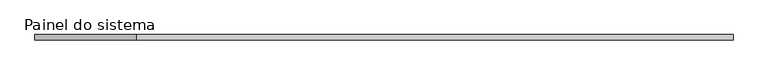
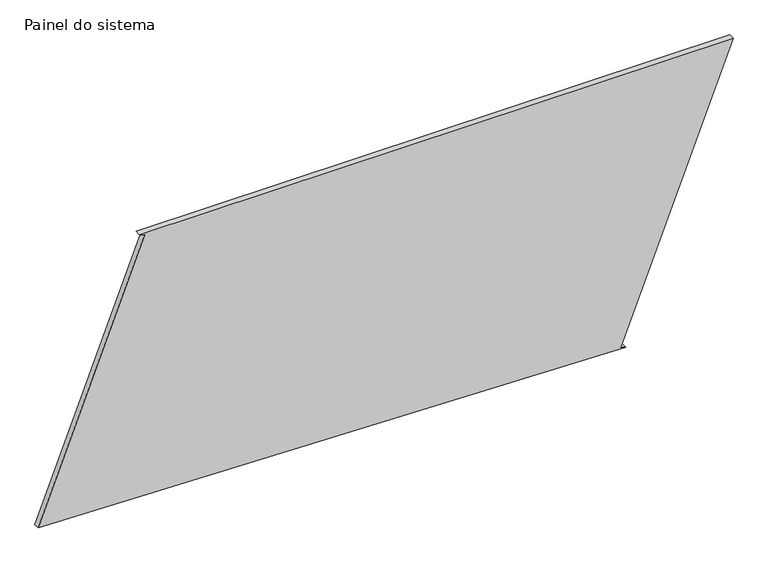
"""IFC4 building model written with IfcOpenShell, lengths in millimetres: plate geometry, Painel do sistema : Envidraçado."""

import ifcopenshell
import ifcopenshell.guid

model = None  # the IFC model being written
_history = None  # IfcOwnerHistory: only IFC2X3 demands one
_inside = {}  # id of a spatial element -> (the spatial element, [elements in it])
_under = {}  # id of a project, library or spatial element -> (it, [spatial elements below it])
_declared = {}  # id of a project -> (the project, [libraries it declares])
_typed = {}  # id of a type object -> (the type object, [elements of that type])
_made_of = {}  # id of a material, layer set ... -> (it, [elements and type objects made of it])


def new_model(schema):
    """Start an empty IFC model of exactly this schema.

    Asked for "IFC4X3", IfcOpenShell would pick the latest addendum, in which some entities
    have other attributes; the version numbers below select the first issue.
    IFC2X3 requires an IfcOwnerHistory on every rooted entity: one is made here for all.
    """
    global model, _history
    if schema == "IFC4X3":
        model = ifcopenshell.file(schema_version=(4, 3, 0, 0))
    else:
        model = ifcopenshell.file(schema=schema)
    _inside.clear()
    _under.clear()
    _declared.clear()
    _typed.clear()
    _made_of.clear()
    _history = None
    if model.schema == "IFC2X3":
        org = make("IfcOrganization", Name="unknown")
        user = make(
            "IfcPersonAndOrganization",
            ThePerson=make("IfcPerson", FamilyName="unknown"),
            TheOrganization=org,
        )
        app = make(
            "IfcApplication",
            ApplicationDeveloper=org,
            Version="unknown",
            ApplicationFullName="unknown",
            ApplicationIdentifier="unknown",
        )
        _history = make(
            "IfcOwnerHistory",
            OwningUser=user,
            OwningApplication=app,
            ChangeAction="ADDED",
            CreationDate=0,
        )
    return model


def make(cls, **values):
    """One entity of the class cls with the attributes given. An attribute that is None is left unset."""
    return model.create_entity(
        cls, **{name: value for name, value in values.items() if value is not None}
    )


def rooted(cls, **values):
    """An entity with a GlobalId (a new one), such as an element, a storey or a relation."""
    return make(cls, GlobalId=ifcopenshell.guid.new(), OwnerHistory=_history, **values)


def si_unit(unit_type, name, prefix=None):
    """IfcSIUnit, for example si_unit("LENGTHUNIT", "METRE", prefix="MILLI")."""
    return make("IfcSIUnit", UnitType=unit_type, Prefix=prefix, Name=name)


def assignment(units):
    """IfcUnitAssignment: the units of a project."""
    return None if units is None else make("IfcUnitAssignment", Units=units)


def point(xyz):
    """IfcCartesianPoint."""
    return None if xyz is None else make("IfcCartesianPoint", Coordinates=xyz)


def direction(xyz):
    """IfcDirection."""
    return None if xyz is None else make("IfcDirection", DirectionRatios=xyz)


def frame(location, z_axis=None, x_axis=None):
    """IfcAxis2Placement3D, a coordinate frame: its origin and axes. An axis left out is left unset."""
    return make(
        "IfcAxis2Placement3D",
        Location=point(location),
        Axis=direction(z_axis),
        RefDirection=direction(x_axis),
    )


def origin():
    """The frame at (0, 0, 0) with its axes left unset."""
    return frame((0.0, 0.0, 0.0))


def place(relative_to, where):
    """IfcLocalPlacement: puts the frame where relative to a parent placement (None: the world)."""
    return make(
        "IfcLocalPlacement", PlacementRelTo=relative_to, RelativePlacement=where
    )


def context(
    kind, dimensions, precision=None, world=None, true_north=None, identifier=None
):
    """IfcGeometricRepresentationContext, for example the 3D "Model" context."""
    return make(
        "IfcGeometricRepresentationContext",
        ContextIdentifier=identifier,
        ContextType=kind,
        CoordinateSpaceDimension=dimensions,
        Precision=precision,
        WorldCoordinateSystem=world,
        TrueNorth=true_north,
    )


def project(units=None, contexts=None):
    """IfcProject with its units and contexts."""
    return rooted(
        "IfcProject",
        Name="project",
        RepresentationContexts=contexts,
        UnitsInContext=assignment(units),
    )


def spatial(cls, under=None, at=None, **own):
    """A site, building, storey or space (cls), placed at a placement, below another one or the project."""
    s = rooted(cls, ObjectPlacement=at, **own)
    if under is not None:
        _under.setdefault(under.id(), (under, []))[1].append(s)
    return s


def polyline(points):
    """IfcPolyline through the points."""
    return make("IfcPolyline", Points=[point(p) for p in points])


def outline(outer, holes=None, kind="AREA"):
    """IfcArbitraryClosedProfileDef: a profile drawn as a closed curve; with holes, ...WithVoids."""
    if holes is None:
        return make("IfcArbitraryClosedProfileDef", ProfileType=kind, OuterCurve=outer)
    return make(
        "IfcArbitraryProfileDefWithVoids",
        ProfileType=kind,
        OuterCurve=outer,
        InnerCurves=holes,
    )


def extrude(swept, where, along, depth):
    """IfcExtrudedAreaSolid: the profile swept, set in the frame where, extruded along a direction by depth."""
    return make(
        "IfcExtrudedAreaSolid",
        SweptArea=swept,
        Position=where,
        ExtrudedDirection=direction(along),
        Depth=depth,
    )


def shape(context_of_items, identifier, shape_type, items):
    """IfcShapeRepresentation: the items that make up one representation, for example the "Body"."""
    return make(
        "IfcShapeRepresentation",
        ContextOfItems=context_of_items,
        RepresentationIdentifier=identifier,
        RepresentationType=shape_type,
        Items=items,
    )


def source(mapping_origin, context_of_items, identifier, shape_type, items):
    """IfcRepresentationMap: a shape defined once, which mapped items show again and again."""
    return make(
        "IfcRepresentationMap",
        MappingOrigin=mapping_origin,
        MappedRepresentation=shape(context_of_items, identifier, shape_type, items),
    )


def transform(
    local_origin,
    x_axis=None,
    y_axis=None,
    z_axis=None,
    scale=None,
    scale2=None,
    scale3=None,
    uniform=True,
):
    """IfcCartesianTransformationOperator3D, or its non-uniform kind. x_axis, y_axis, z_axis: its Axis1, 2, 3."""
    if uniform:
        return make(
            "IfcCartesianTransformationOperator3D",
            Axis1=direction(x_axis),
            Axis2=direction(y_axis),
            LocalOrigin=point(local_origin),
            Scale=scale,
            Axis3=direction(z_axis),
        )
    return make(
        "IfcCartesianTransformationOperator3DnonUniform",
        Axis1=direction(x_axis),
        Axis2=direction(y_axis),
        LocalOrigin=point(local_origin),
        Scale=scale,
        Axis3=direction(z_axis),
        Scale2=scale2,
        Scale3=scale3,
    )


def mapped(mapping_source, mapping_target):
    """IfcMappedItem: shows the shape of a source again, moved by a transform."""
    return make(
        "IfcMappedItem", MappingSource=mapping_source, MappingTarget=mapping_target
    )


def made_of(thing, what):
    """Note that an element or type object is made of a material, layer set ...; save() writes the relation."""
    if what is not None:
        _made_of.setdefault(what.id(), (what, []))[1].append(thing)
    return thing


def element(
    cls,
    number,
    at=None,
    inside=None,
    cuts=None,
    type_object=None,
    material=None,
    context=None,
    identifier="Body",
    shape_type=None,
    held_by="IfcProductDefinitionShape",
    body=None,
    shapes=None,
    **own,
):
    """One element of the class cls, such as IfcWall. Its Tag is "e" and its number.

    at: its placement. inside: the storey or other place that contains it. cuts: it is an
    opening in that element (IfcRelVoidsElement). A single representation is given by context,
    identifier, shape_type and body (its items); several are given by shapes. held_by: the class
    of the entity that holds the representations. save() writes the other relations.
    """
    e = rooted(cls, Tag="e%d" % number, ObjectPlacement=at, **own)
    if body is not None:
        shapes = [shape(context, identifier, shape_type, body)]
    if shapes is not None:
        e.Representation = make(held_by, Representations=shapes)
    if inside is not None:
        _inside.setdefault(inside.id(), (inside, []))[1].append(e)
    if cuts is not None:
        rooted(
            "IfcRelVoidsElement", RelatingBuildingElement=cuts, RelatedOpeningElement=e
        )
    if type_object is not None:
        _typed.setdefault(type_object.id(), (type_object, []))[1].append(e)
    return made_of(e, material)


def aggregate(whole, parts):
    """IfcRelAggregates: a whole, such as a stair, and the parts it consists of."""
    return rooted("IfcRelAggregates", RelatingObject=whole, RelatedObjects=parts)


def save(model, path):
    """Write the relations noted so far, then the file.

    IfcRelAggregates (storeys below a building ...), IfcRelContainedInSpatialStructure (elements
    in a storey), IfcRelDefinesByType, IfcRelAssociatesMaterial and IfcRelDeclares: one each for
    every whole, place, type object, material and project.
    """
    for whole, parts in _under.values():
        aggregate(whole, parts)
    for where, things in _inside.values():
        rooted(
            "IfcRelContainedInSpatialStructure",
            RelatedElements=things,
            RelatingStructure=where,
        )
    for kind, things in _typed.values():
        rooted("IfcRelDefinesByType", RelatedObjects=things, RelatingType=kind)
    for what, things in _made_of.values():
        rooted("IfcRelAssociatesMaterial", RelatedObjects=things, RelatingMaterial=what)
    for by, libraries in _declared.values():
        rooted("IfcRelDeclares", RelatingContext=by, RelatedDefinitions=libraries)
    model.write(path)


def painel_do_sistema_89789c02(model_context):
    return source(origin(), model_context, "Body", "SweptSolid", [
        extrude(outline(polyline([(0.0, 1107.0608873), (9.0972802, 1083.7748509), (1333.7866514, 1601.2983243), (1333.7866514, -1133.8482806), (1324.6893712, -1110.5622442), (68.5668902, -1601.2983243), (0.0, 1107.0608873)])), frame((0.0, 24.5, 0.0), z_axis=(0.0, 1.0, 0.0), x_axis=(0.0, 0.0, 1.0)), (0.0, 0.0, 1.0), 25.0),
    ])


if __name__ == "__main__":
    model = new_model("IFC4")
    model_context = context("Model", 3, world=origin())
    ifc_project = project(units=[si_unit("LENGTHUNIT", "METRE", prefix="MILLI")], contexts=[model_context])
    site = spatial("IfcSite", under=ifc_project)
    building = spatial("IfcBuilding", under=site)
    placement = place(None, origin())
    painel_do_sistema_shape = painel_do_sistema_89789c02(model_context)
    element("IfcPlate", 1, ObjectType="Painel do sistema : Envidraçado", at=placement, inside=building, context=model_context, shape_type="MappedRepresentation", body=[
        mapped(painel_do_sistema_shape, transform((0.0, 0.0, 0.0), x_axis=(1.0, 0.0, 0.0), y_axis=(0.0, 1.0, 0.0), z_axis=(0.0, 0.0, 1.0))),
    ])
    save(model, "model.ifc")

# Revit data of these elements
# Type "Painel do sistema : Envidraçado"
#   Construction Type Id = "GSP4R"
#   Analytic Construction = "Vidraça única Pilkington 1/8 pol"
#   Visual Light Transmittance = 0.9
#   Solar Heat Gain Coefficient = 0.86
#   Heat Transfer Coefficient (U) = 6.7069 W/(m²·K)
# Element 1 (IfcPlate, "Painel do sistema : Envidraçado")
#   Materials on its faces: "Vidro"
# Materials
#   "Vidro": class "Vidro", colour RGB 0 128 192, transparency 0.9, Description = "Vidro de sílica", Cost = 0
